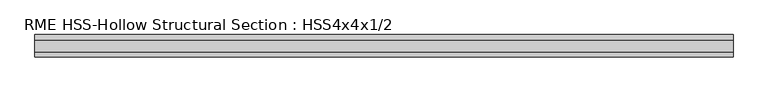
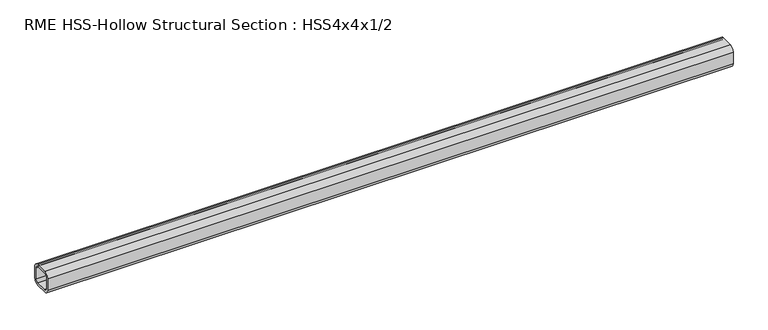
"""IFC4 building model written with IfcOpenShell, lengths in millimetres: member geometry, RME HSS-Hollow Structural Section : HSS4x4x1/2."""

from ifc_helpers import new_model, si_unit, point, frame, frame_2d, origin, place, context, project, spatial, polyline, circle_curve, trimmed, segment, composite_curve, outline, extrude, source, transform, mapped, element, save


def rme_hss_hollow_structural_section_hss4x4x1_2_ac98842f(model_context):
    return source(origin(), model_context, "Body", "SweptSolid", [
        extrude(outline(composite_curve([segment(polyline([(50.8, 27.178), (50.8, -27.178)]), True, "CONTINUOUS"), segment(trimmed(circle_curve(frame_2d((27.178, -27.178)), 23.622), [point((50.8, -27.178))], [point((27.178, -50.8))], False, "CARTESIAN"), True, "CONTINUOUS"), segment(polyline([(27.178, -50.8), (-27.178, -50.8)]), True, "CONTINUOUS"), segment(trimmed(circle_curve(frame_2d((-27.178, -27.178)), 23.622), [point((-27.178, -50.8))], [point((-50.8, -27.178))], False, "CARTESIAN"), True, "CONTINUOUS"), segment(polyline([(-50.8, -27.178), (-50.8, 27.178)]), True, "CONTINUOUS"), segment(trimmed(circle_curve(frame_2d((-27.178, 27.178)), 23.622), [point((-50.8, 27.178))], [point((-27.178, 50.8))], False, "CARTESIAN"), True, "CONTINUOUS"), segment(polyline([(-27.178, 50.8), (27.178, 50.8)]), True, "CONTINUOUS"), segment(trimmed(circle_curve(frame_2d((27.178, 27.178)), 23.622), [point((27.178, 50.8))], [point((50.8, 27.178))], False, "CARTESIAN"), True, "CONTINUOUS")], self_intersect=False), holes=[composite_curve([segment(trimmed(circle_curve(frame_2d((-27.178, 27.178)), 11.811), [point((-27.178, 38.989))], [point((-38.989, 27.178))], True, "CARTESIAN"), True, "CONTINUOUS"), segment(polyline([(-38.989, 27.178), (-38.989, -27.178)]), True, "CONTINUOUS"), segment(trimmed(circle_curve(frame_2d((-27.178, -27.178)), 11.811), [point((-38.989, -27.178))], [point((-27.178, -38.989))], True, "CARTESIAN"), True, "CONTINUOUS"), segment(polyline([(-27.178, -38.989), (27.178, -38.989)]), True, "CONTINUOUS"), segment(trimmed(circle_curve(frame_2d((27.178, -27.178)), 11.811), [point((27.178, -38.989))], [point((38.989, -27.178))], True, "CARTESIAN"), True, "CONTINUOUS"), segment(polyline([(38.989, -27.178), (38.989, 27.178)]), True, "CONTINUOUS"), segment(trimmed(circle_curve(frame_2d((27.178, 27.178)), 11.811), [point((38.989, 27.178))], [point((27.178, 38.989))], True, "CARTESIAN"), True, "CONTINUOUS"), segment(polyline([(27.178, 38.989), (-27.178, 38.989)]), True, "CONTINUOUS")], self_intersect=False)]), frame((-1486.8968239, 0.0, 0.0), z_axis=(1.0, 0.0, 0.0), x_axis=(0.0, 1.0, 0.0)), (0.0, 0.0, 1.0), 3165.1669952),
    ])


if __name__ == "__main__":
    model = new_model("IFC4")
    model_context = context("Model", 3, world=origin())
    ifc_project = project(units=[si_unit("LENGTHUNIT", "METRE", prefix="MILLI")], contexts=[model_context])
    site = spatial("IfcSite", under=ifc_project)
    building = spatial("IfcBuilding", under=site)
    placement = place(None, origin())
    rme_hss_hollow_structural_section_hss4x4x1_2_shape = rme_hss_hollow_structural_section_hss4x4x1_2_ac98842f(model_context)
    element("IfcMember", 1, ObjectType="RME HSS-Hollow Structural Section : HSS4x4x1/2", at=placement, inside=building, context=model_context, shape_type="MappedRepresentation", body=[
        mapped(rme_hss_hollow_structural_section_hss4x4x1_2_shape, transform((0.0, 0.0, 0.0), x_axis=(1.0, 0.0, 0.0), y_axis=(0.0, 1.0, 0.0), z_axis=(0.0, 0.0, 1.0))),
    ])
    save(model, "model.ifc")

# Revit data of these elements
# Type "RME HSS-Hollow Structural Section : HSS4x4x1/2"
#   Nominal Size = "HSS6x4"
#   Assembly Code = "B10"
#   Shape = "Square"
#   W = 21.5
#   Start Extension Calculation [instance default] = 10' - 0"
#   Start Extension [instance default] = -0' - 0 1/2"
#   End Extension Calculation [instance default] = 10' - 0"
#   End Extension [instance default] = -0' - 0 1/2"
#   Ht = 0' - 4"
#   Length [instance default] = 5' - 0"
#   b = 0' - 4"
#   kr = 0' - 0.93"
#   t = 0' - 0.465"
#   A = 0.0418056 SF
#   Structural Material [instance default] = Metal - Steel - ASTM A500 - Grade B - Rectangular and Square
# Element 1 (IfcMember, "RME HSS-Hollow Structural Section : HSS4x4x1/2")
#   Length = 11' - 7.34508"
#   Structural Material = Metal - Steel - ASTM A992
#   Materials on its faces: "Metal - Steel - ASTM A992"
# Materials
#   "Metal - Steel - ASTM A500 - Grade B - Rectangular and Square": class "Metal", colour RGB 255 128 0, transparency 0
#   "Metal - Steel - ASTM A992": class "Metal", colour RGB 255 128 0, transparency 0
